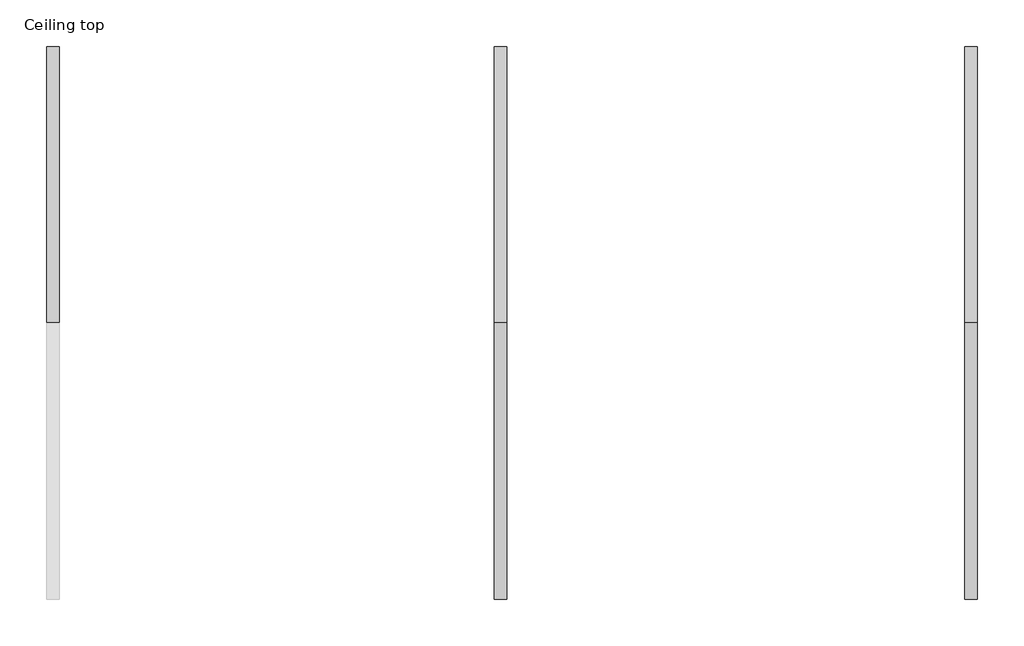
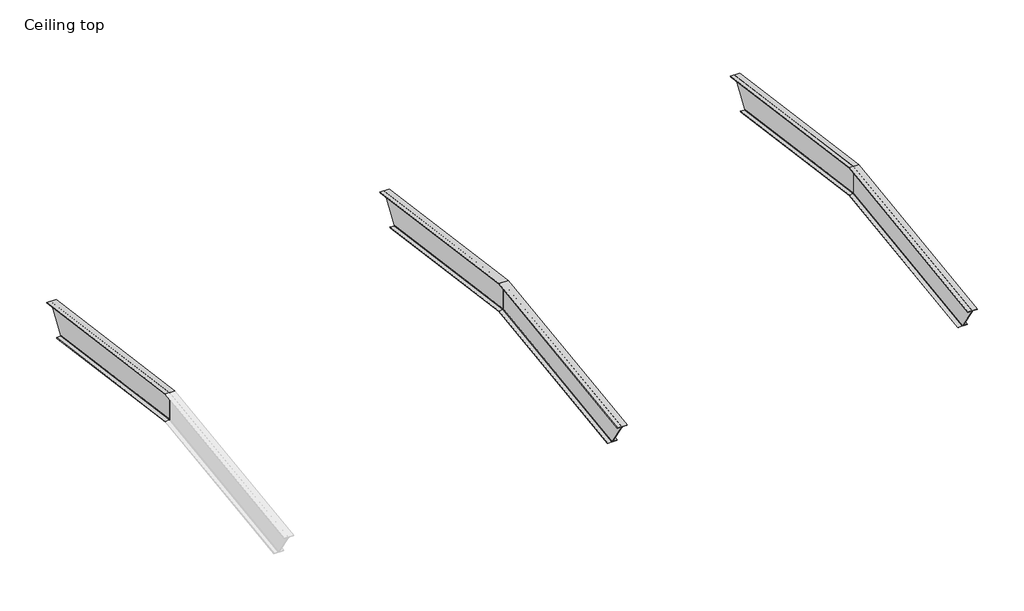
# One storey, part 2 of 2: 5 beams.
"""IFC4 building model written with IfcOpenShell, lengths in millimetres."""

from ifc_helpers import new_model, si_unit, frame, origin, place, context, project, spatial, polyline, ellipse_curve, element, save
from ifc_brep_helpers import plane_surface, revolved_surface, advanced_brep

model = new_model("IFC4")

# Units and contexts
model_context = context("Model", 3, world=origin())
ifc_project = project(units=[si_unit("LENGTHUNIT", "METRE", prefix="MILLI")], contexts=[model_context])

# Site, building, storey
site = spatial("IfcSite", under=ifc_project)
building = spatial("IfcBuilding", under=site)
storey = spatial("IfcBuildingStorey", under=building, Name="Ceiling top", Elevation=4718.05)

# Beams
placement = place(None, origin())
element("IfcBeam", 1, ObjectType="W Shapes : W 6X18.5", at=placement, inside=storey, context=model_context, shape_type="AdvancedBrep", body=[
    advanced_brep(
    [(28967.3280052, 7113.2615366, 4727.7884676), (29032.9870052, 7113.2615366, 4727.7884676), (29032.9870052, 10139.0601337, 4314.3781499), (28967.3280052, 10139.0601337, 4314.3781499), (28959.7080052, 7113.2615366, 4735.4792613), (28959.7080052, 10143.6843616, 4321.4371423), (28959.7080052, 7113.2615366, 5174.8799434), (28959.7080052, 10407.8819145, 4724.7409096), (28967.3280052, 7113.2615366, 5182.5707371), (28967.3280052, 10412.5061424, 4731.799902), (29032.9870052, 7113.2615366, 5182.5707371), (29032.9870052, 10412.5061424, 4731.799902), (29032.9870052, 7113.2615366, 5192.3124092), (29032.9870052, 10418.3634977, 4740.7412924), (28880.5870052, 7113.2615366, 5192.3124092), (28880.5870052, 10418.3634977, 4740.7412924), (28880.5870052, 7113.2615366, 5182.5707371), (28880.5870052, 10412.5061424, 4731.799902), (28946.2460052, 7113.2615366, 5182.5707371), (28946.2460052, 10412.5061424, 4731.799902), (28953.8660052, 7113.2615366, 5174.8799434), (28953.8660052, 10407.8819145, 4724.7409096), (28953.8660052, 7113.2615366, 4735.4792613), (28953.8660052, 10143.6843616, 4321.4371423), (28946.2460052, 7113.2615366, 4727.7884676), (28946.2460052, 10139.0601337, 4314.3781499), (28880.5870052, 7113.2615366, 4727.7884676), (28880.5870052, 10139.0601337, 4314.3781499), (28880.5870052, 7113.2615366, 4718.0467955), (28880.5870052, 10133.2027784, 4305.4367595), (29032.9870052, 7113.2615366, 4718.0467955), (29032.9870052, 10133.2027784, 4305.4367595)],
    [
        (0, 1),
        (1, 2),
        (2, 3),
        (3, 0),
        (4, 0, ellipse_curve(frame((28967.3280052, 7113.2615366, 4735.4792613), z_axis=(0.0, -1.0, 0.0), x_axis=(0.0, 0.0, -1.0)), 7.6907937, 7.62)),
        (3, 5, ellipse_curve(frame((28967.3280052, 10143.6843616, 4321.4371423), z_axis=(0.0, 0.836495308057375, -0.5479740866117643), x_axis=(0.0, 0.547974086611764, 0.8364953080573752)), 8.4387711, 7.62)),
        (5, 4),
        (6, 4),
        (5, 7),
        (7, 6),
        (8, 6, ellipse_curve(frame((28967.3280052, 7113.2615366, 5174.8799434), z_axis=(0.0, -1.0, 0.0), x_axis=(0.0, 0.0, -1.0)), 7.6907937, 7.62)),
        (7, 9, ellipse_curve(frame((28967.3280052, 10407.8819145, 4724.7409096), z_axis=(0.0, 0.836495308057375, -0.5479740866117643), x_axis=(0.0, 0.547974086611764, 0.8364953080573752)), 8.4387711, 7.62)),
        (9, 8),
        (10, 8),
        (9, 11),
        (11, 10),
        (12, 10),
        (11, 13),
        (13, 12),
        (14, 12),
        (13, 15),
        (15, 14),
        (16, 14),
        (15, 17),
        (17, 16),
        (18, 16),
        (17, 19),
        (19, 18),
        (20, 18, ellipse_curve(frame((28946.2460052, 7113.2615366, 5174.8799434), z_axis=(0.0, -1.0, 0.0), x_axis=(0.0, 0.0, -1.0)), 7.6907937, 7.62)),
        (19, 21, ellipse_curve(frame((28946.2460052, 10407.8819145, 4724.7409096), z_axis=(0.0, 0.836495308057375, -0.5479740866117643), x_axis=(0.0, 0.547974086611764, 0.8364953080573752)), 8.4387711, 7.62)),
        (21, 20),
        (22, 20),
        (21, 23),
        (23, 22),
        (24, 22, ellipse_curve(frame((28946.2460052, 7113.2615366, 4735.4792613), z_axis=(0.0, -1.0, 0.0), x_axis=(0.0, 0.0, -1.0)), 7.6907937, 7.62)),
        (23, 25, ellipse_curve(frame((28946.2460052, 10143.6843616, 4321.4371423), z_axis=(0.0, 0.836495308057375, -0.5479740866117643), x_axis=(0.0, 0.547974086611764, 0.8364953080573752)), 8.4387711, 7.62)),
        (25, 24),
        (26, 24),
        (25, 27),
        (27, 26),
        (28, 26),
        (27, 29),
        (29, 28),
        (30, 28),
        (29, 31),
        (31, 30),
        (1, 30),
        (31, 2),
    ],
    [
        plane_surface(frame((29032.9870052, 7050.9569516, 4736.3010494), z_axis=(0.0, 0.1353708330841357, 0.9907950027882191), x_axis=(0.0, 0.9907950027882191, -0.1353708330841357))),
        revolved_surface(polyline([(28959.708005200002, 10147.277063747912, 4320.946276885532), (28959.708005200002, 7112.230010863546, 4735.620197164001)]), (28967.3280052, 7051.9884774, 4743.8509074), (0.0, 0.9907950027882191, -0.1353708330841357)),
        plane_surface(frame((28959.7080052, 7051.9884774, 4743.8509074), z_axis=(1.0, 0.0, 0.0), x_axis=(0.0, 0.9907950027882191, -0.1353708330841357))),
        revolved_surface(polyline([(28959.708005200002, 10411.474616650441, 4724.25004406808), (28959.708005200002, 7112.230010852571, 5175.020879183669)]), (28967.3280052, 7110.9229818, 5175.1994566), (0.0, 0.9907950027882191, -0.1353708330841357)),
        plane_surface(frame((28967.3280052, 7111.9545075, 5182.7493145), z_axis=(0.0, -0.1353708330841357, -0.9907950027882191), x_axis=(0.0, 0.9907950027882191, -0.1353708330841357))),
        plane_surface(frame((29032.9870052, 7111.9545075, 5182.7493145), z_axis=(1.0, 0.0, 0.0), x_axis=(0.0, 0.9907950027882191, -0.1353708330841357))),
        plane_surface(frame((29032.9870052, 7113.2611068, 5192.3124679), z_axis=(0.0, 0.1353708330841357, 0.9907950027882191), x_axis=(0.0, 0.9907950027882191, -0.1353708330841357))),
        plane_surface(frame((28880.5870052, 7113.2611068, 5192.3124679), z_axis=(-1.0, 0.0, 0.0), x_axis=(0.0, 0.9907950027882191, -0.1353708330841357))),
        plane_surface(frame((28880.5870052, 7111.9545075, 5182.7493145), z_axis=(0.0, -0.1353708330841357, -0.9907950027882191), x_axis=(0.0, 0.9907950027882191, -0.1353708330841357))),
        revolved_surface(polyline([(28938.6260052, 10411.474616650441, 4724.25004406808), (28938.6260052, 7112.230010852571, 5175.020879183669)]), (28946.2460052, 7110.9229818, 5175.1994566), (0.0, 0.9907950027882191, -0.1353708330841357)),
        plane_surface(frame((28953.8660052, 7110.9229818, 5175.1994566), z_axis=(-1.0, 0.0, 0.0), x_axis=(0.0, 0.9907950027882191, -0.1353708330841357))),
        revolved_surface(polyline([(28938.6260052, 10147.277063747912, 4320.946276885532), (28938.6260052, 7112.230010863546, 4735.620197164001)]), (28946.2460052, 7051.9884774, 4743.8509074), (0.0, 0.9907950027882191, -0.1353708330841357)),
        plane_surface(frame((28946.2460052, 7050.9569516, 4736.3010494), z_axis=(0.0, 0.1353708330841357, 0.9907950027882191), x_axis=(0.0, 0.9907950027882191, -0.1353708330841357))),
        plane_surface(frame((28880.5870052, 7050.9569516, 4736.3010494), z_axis=(-1.0, 0.0, 0.0), x_axis=(0.0, 0.9907950027882191, -0.1353708330841357))),
        plane_surface(frame((28880.5870052, 7049.6503524, 4726.7378961), z_axis=(0.0, -0.1353708330841357, -0.9907950027882191), x_axis=(0.0, 0.9907950027882191, -0.1353708330841357))),
        plane_surface(frame((29032.9870052, 7049.6503524, 4726.7378961), z_axis=(1.0, 0.0, 0.0), x_axis=(0.0, 0.9907950027882191, -0.1353708330841357))),
        plane_surface(frame((28956.7905771, 10418.3654245, 4740.7442336), z_axis=(0.0, 0.836495308057375, -0.5479740866117643), x_axis=(1.0, 0.0, 0.0))),
        plane_surface(frame((28956.7905771, 7113.2615366, 5192.3156137), z_axis=(0.0, -1.0, 0.0), x_axis=(0.0, 0.0, 1.0))),
    ],
    [
        (0, [[1, 2, 3, 4]]),
        (1, [[5, -4, 6, 7]]),
        (2, [[8, -7, 9, 10]]),
        (3, [[11, -10, 12, 13]]),
        (4, [[14, -13, 15, 16]]),
        (5, [[17, -16, 18, 19]]),
        (6, [[20, -19, 21, 22]]),
        (7, [[23, -22, 24, 25]]),
        (8, [[26, -25, 27, 28]]),
        (9, [[29, -28, 30, 31]]),
        (10, [[32, -31, 33, 34]]),
        (11, [[35, -34, 36, 37]]),
        (12, [[38, -37, 39, 40]]),
        (13, [[41, -40, 42, 43]]),
        (14, [[44, -43, 45, 46]]),
        (15, [[47, -46, 48, -2]]),
        (16, [[-48, -45, -42, -39, -36, -33, -30, -27, -24, -21, -18, -15, -12, -9, -6, -3]]),
        (17, [[-1, -5, -8, -11, -14, -17, -20, -23, -26, -29, -32, -35, -38, -41, -44, -47]]),
    ],
),
])
element("IfcBeam", 2, ObjectType="W Shapes : W 6X18.5", at=placement, inside=storey, context=model_context, shape_type="AdvancedBrep", body=[
    advanced_brep(
    [(28967.3280052, 4087.4629396, 4314.3781499), (29032.9870052, 4087.4629396, 4314.3781499), (29032.9870052, 7113.2615366, 4727.7884676), (28967.3280052, 7113.2615366, 4727.7884676), (28959.7080052, 4082.8387117, 4321.4371423), (28959.7080052, 7113.2615366, 4735.4792613), (28959.7080052, 3818.6411587, 4724.7409096), (28959.7080052, 7113.2615366, 5174.8799434), (28967.3280052, 3814.0169308, 4731.799902), (28967.3280052, 7113.2615366, 5182.5707371), (29032.9870052, 3814.0169308, 4731.799902), (29032.9870052, 7113.2615366, 5182.5707371), (29032.9870052, 3808.1595755, 4740.7412924), (29032.9870052, 7113.2615366, 5192.3124092), (28880.5870052, 3808.1595755, 4740.7412924), (28880.5870052, 7113.2615366, 5192.3124092), (28880.5870052, 3814.0169308, 4731.799902), (28880.5870052, 7113.2615366, 5182.5707371), (28946.2460052, 3814.0169308, 4731.799902), (28946.2460052, 7113.2615366, 5182.5707371), (28953.8660052, 3818.6411587, 4724.7409096), (28953.8660052, 7113.2615366, 5174.8799434), (28953.8660052, 4082.8387117, 4321.4371423), (28953.8660052, 7113.2615366, 4735.4792613), (28946.2460052, 4087.4629396, 4314.3781499), (28946.2460052, 7113.2615366, 4727.7884676), (28880.5870052, 4087.4629396, 4314.3781499), (28880.5870052, 7113.2615366, 4727.7884676), (28880.5870052, 4093.3202949, 4305.4367595), (28880.5870052, 7113.2615366, 4718.0467955), (29032.9870052, 4093.3202949, 4305.4367595), (29032.9870052, 7113.2615366, 4718.0467955)],
    [
        (0, 1),
        (1, 2),
        (2, 3),
        (3, 0),
        (4, 0, ellipse_curve(frame((28967.3280052, 4082.8387117, 4321.4371423), z_axis=(0.0, -0.8364953080573767, -0.5479740866117618), x_axis=(0.0, 0.5479740866117613, -0.8364953080573769)), 8.4387711, 7.62)),
        (3, 5, ellipse_curve(frame((28967.3280052, 7113.2615366, 4735.4792613), z_axis=(0.0, 1.0, 0.0), x_axis=(0.0, 0.0, 1.0)), 7.6907937, 7.62)),
        (5, 4),
        (6, 4),
        (5, 7),
        (7, 6),
        (8, 6, ellipse_curve(frame((28967.3280052, 3818.6411587, 4724.7409096), z_axis=(0.0, -0.8364953080573767, -0.5479740866117618), x_axis=(0.0, 0.5479740866117613, -0.8364953080573769)), 8.4387711, 7.62)),
        (7, 9, ellipse_curve(frame((28967.3280052, 7113.2615366, 5174.8799434), z_axis=(0.0, 1.0, 0.0), x_axis=(0.0, 0.0, 1.0)), 7.6907937, 7.62)),
        (9, 8),
        (10, 8),
        (9, 11),
        (11, 10),
        (12, 10),
        (11, 13),
        (13, 12),
        (14, 12),
        (13, 15),
        (15, 14),
        (16, 14),
        (15, 17),
        (17, 16),
        (18, 16),
        (17, 19),
        (19, 18),
        (20, 18, ellipse_curve(frame((28946.2460052, 3818.6411587, 4724.7409096), z_axis=(0.0, -0.8364953080573767, -0.5479740866117618), x_axis=(0.0, 0.5479740866117613, -0.8364953080573769)), 8.4387711, 7.62)),
        (19, 21, ellipse_curve(frame((28946.2460052, 7113.2615366, 5174.8799434), z_axis=(0.0, 1.0, 0.0), x_axis=(0.0, 0.0, 1.0)), 7.6907937, 7.62)),
        (21, 20),
        (22, 20),
        (21, 23),
        (23, 22),
        (24, 22, ellipse_curve(frame((28946.2460052, 4082.8387117, 4321.4371423), z_axis=(0.0, -0.8364953080573767, -0.5479740866117618), x_axis=(0.0, 0.5479740866117613, -0.8364953080573769)), 8.4387711, 7.62)),
        (23, 25, ellipse_curve(frame((28946.2460052, 7113.2615366, 4735.4792613), z_axis=(0.0, 1.0, 0.0), x_axis=(0.0, 0.0, 1.0)), 7.6907937, 7.62)),
        (25, 24),
        (26, 24),
        (25, 27),
        (27, 26),
        (28, 26),
        (27, 29),
        (29, 28),
        (30, 28),
        (29, 31),
        (31, 30),
        (1, 30),
        (31, 2),
    ],
    [
        plane_surface(frame((29032.9870052, 3870.4622337, 4284.7296694), z_axis=(0.0, -0.13537083308413533, 0.9907950027882192), x_axis=(0.0, 0.9907950027882192, 0.13537083308413533))),
        revolved_surface(polyline([(28959.708005200002, 7114.293062347846, 4735.620197080616), (28959.708005200002, 4079.246009561649, 4320.946276815561)]), (28967.3280052, 3869.430708, 4292.2795273), (0.0, 0.9907950027882191, 0.1353708330841353)),
        plane_surface(frame((28959.7080052, 3869.430708, 4292.2795273), z_axis=(1.0, 0.0, 0.0), x_axis=(0.0, 0.9907950027882192, 0.13537083308413533))),
        revolved_surface(polyline([(28959.708005200002, 7114.293062345409, 5175.020879198452), (28959.708005200002, 3815.0484565475394, 4724.2500440828635)]), (28967.3280052, 3810.4962036, 4723.6280766), (0.0, 0.9907950027882191, 0.1353708330841353)),
        plane_surface(frame((28967.3280052, 3809.4646778, 4731.1779345), z_axis=(0.0, 0.13537083308413533, -0.9907950027882192), x_axis=(0.0, 0.9907950027882192, 0.13537083308413533))),
        plane_surface(frame((29032.9870052, 3809.4646778, 4731.1779345), z_axis=(1.0, 0.0, 0.0), x_axis=(0.0, 0.9907950027882192, 0.13537083308413533))),
        plane_surface(frame((29032.9870052, 3808.1580786, 4740.7410879), z_axis=(0.0, -0.13537083308413533, 0.9907950027882192), x_axis=(0.0, 0.9907950027882192, 0.13537083308413533))),
        plane_surface(frame((28880.5870052, 3808.1580786, 4740.7410879), z_axis=(-1.0, 0.0, 0.0), x_axis=(0.0, 0.9907950027882192, 0.13537083308413533))),
        plane_surface(frame((28880.5870052, 3809.4646778, 4731.1779345), z_axis=(0.0, 0.13537083308413533, -0.9907950027882192), x_axis=(0.0, 0.9907950027882192, 0.13537083308413533))),
        revolved_surface(polyline([(28938.6260052, 7114.293062345409, 5175.020879198452), (28938.6260052, 3815.0484565475394, 4724.2500440828635)]), (28946.2460052, 3810.4962036, 4723.6280766), (0.0, 0.9907950027882191, 0.1353708330841353)),
        plane_surface(frame((28953.8660052, 3810.4962036, 4723.6280766), z_axis=(-1.0, 0.0, 0.0), x_axis=(0.0, 0.9907950027882192, 0.13537083308413533))),
        revolved_surface(polyline([(28938.6260052, 7114.293062347846, 4735.620197080616), (28938.6260052, 4079.246009561649, 4320.946276815561)]), (28946.2460052, 3869.430708, 4292.2795273), (0.0, 0.9907950027882191, 0.1353708330841353)),
        plane_surface(frame((28946.2460052, 3870.4622337, 4284.7296694), z_axis=(0.0, -0.13537083308413533, 0.9907950027882192), x_axis=(0.0, 0.9907950027882192, 0.13537083308413533))),
        plane_surface(frame((28880.5870052, 3870.4622337, 4284.7296694), z_axis=(-1.0, 0.0, 0.0), x_axis=(0.0, 0.9907950027882192, 0.13537083308413533))),
        plane_surface(frame((28880.5870052, 3871.768833, 4275.166516), z_axis=(0.0, 0.13537083308413533, -0.9907950027882192), x_axis=(0.0, 0.9907950027882192, 0.13537083308413533))),
        plane_surface(frame((29032.9870052, 3871.768833, 4275.166516), z_axis=(1.0, 0.0, 0.0), x_axis=(0.0, 0.9907950027882192, 0.13537083308413533))),
        plane_surface(frame((28956.7905771, 7113.2615366, 5192.3156137), z_axis=(0.0, 1.0, 0.0), x_axis=(0.0, 0.0, -1.0))),
        plane_surface(frame((28956.7905771, 4093.3183681, 4305.4397008), z_axis=(0.0, -0.8364953080573767, -0.5479740866117618), x_axis=(1.0, 0.0, 0.0))),
    ],
    [
        (0, [[1, 2, 3, 4]]),
        (1, [[5, -4, 6, 7]]),
        (2, [[8, -7, 9, 10]]),
        (3, [[11, -10, 12, 13]]),
        (4, [[14, -13, 15, 16]]),
        (5, [[17, -16, 18, 19]]),
        (6, [[20, -19, 21, 22]]),
        (7, [[23, -22, 24, 25]]),
        (8, [[26, -25, 27, 28]]),
        (9, [[29, -28, 30, 31]]),
        (10, [[32, -31, 33, 34]]),
        (11, [[35, -34, 36, 37]]),
        (12, [[38, -37, 39, 40]]),
        (13, [[41, -40, 42, 43]]),
        (14, [[44, -43, 45, 46]]),
        (15, [[47, -46, 48, -2]]),
        (16, [[-48, -45, -42, -39, -36, -33, -30, -27, -24, -21, -18, -15, -12, -9, -6, -3]]),
        (17, [[-1, -5, -8, -11, -14, -17, -20, -23, -26, -29, -32, -35, -38, -41, -44, -47]]),
    ],
),
])
element("IfcBeam", 3, ObjectType="W Shapes : W 6X18.5", at=placement, inside=storey, context=model_context, shape_type="AdvancedBrep", body=[
    advanced_brep(
    [(23341.2280052, 7113.2615366, 4727.7884676), (23406.8870052, 7113.2615366, 4727.7884676), (23406.8870052, 10139.0601337, 4314.3781499), (23341.2280052, 10139.0601337, 4314.3781499), (23333.6080052, 7113.2615366, 4735.4792613), (23333.6080052, 10143.6843616, 4321.4371423), (23333.6080052, 7113.2615366, 5174.8799434), (23333.6080052, 10407.8819145, 4724.7409096), (23341.2280052, 7113.2615366, 5182.5707371), (23341.2280052, 10412.5061424, 4731.799902), (23406.8870052, 7113.2615366, 5182.5707371), (23406.8870052, 10412.5061424, 4731.799902), (23406.8870052, 7113.2615366, 5192.3124092), (23406.8870052, 10418.3634977, 4740.7412924), (23254.4870052, 7113.2615366, 5192.3124092), (23254.4870052, 10418.3634977, 4740.7412924), (23254.4870052, 7113.2615366, 5182.5707371), (23254.4870052, 10412.5061424, 4731.799902), (23320.1460052, 7113.2615366, 5182.5707371), (23320.1460052, 10412.5061424, 4731.799902), (23327.7660052, 7113.2615366, 5174.8799434), (23327.7660052, 10407.8819145, 4724.7409096), (23327.7660052, 7113.2615366, 4735.4792613), (23327.7660052, 10143.6843616, 4321.4371423), (23320.1460052, 7113.2615366, 4727.7884676), (23320.1460052, 10139.0601337, 4314.3781499), (23254.4870052, 7113.2615366, 4727.7884676), (23254.4870052, 10139.0601337, 4314.3781499), (23254.4870052, 7113.2615366, 4718.0467955), (23254.4870052, 10133.2027784, 4305.4367595), (23406.8870052, 7113.2615366, 4718.0467955), (23406.8870052, 10133.2027784, 4305.4367595)],
    [
        (0, 1),
        (1, 2),
        (2, 3),
        (3, 0),
        (4, 0, ellipse_curve(frame((23341.2280052, 7113.2615366, 4735.4792613), z_axis=(0.0, -1.0, 0.0), x_axis=(0.0, 0.0, -1.0)), 7.6907937, 7.62)),
        (3, 5, ellipse_curve(frame((23341.2280052, 10143.6843616, 4321.4371423), z_axis=(0.0, 0.836495308057375, -0.5479740866117643), x_axis=(0.0, 0.547974086611764, 0.8364953080573752)), 8.4387711, 7.62)),
        (5, 4),
        (6, 4),
        (5, 7),
        (7, 6),
        (8, 6, ellipse_curve(frame((23341.2280052, 7113.2615366, 5174.8799434), z_axis=(0.0, -1.0, 0.0), x_axis=(0.0, 0.0, -1.0)), 7.6907937, 7.62)),
        (7, 9, ellipse_curve(frame((23341.2280052, 10407.8819145, 4724.7409096), z_axis=(0.0, 0.836495308057375, -0.5479740866117643), x_axis=(0.0, 0.547974086611764, 0.8364953080573752)), 8.4387711, 7.62)),
        (9, 8),
        (10, 8),
        (9, 11),
        (11, 10),
        (12, 10),
        (11, 13),
        (13, 12),
        (14, 12),
        (13, 15),
        (15, 14),
        (16, 14),
        (15, 17),
        (17, 16),
        (18, 16),
        (17, 19),
        (19, 18),
        (20, 18, ellipse_curve(frame((23320.1460052, 7113.2615366, 5174.8799434), z_axis=(0.0, -1.0, 0.0), x_axis=(0.0, 0.0, -1.0)), 7.6907937, 7.62)),
        (19, 21, ellipse_curve(frame((23320.1460052, 10407.8819145, 4724.7409096), z_axis=(0.0, 0.836495308057375, -0.5479740866117643), x_axis=(0.0, 0.547974086611764, 0.8364953080573752)), 8.4387711, 7.62)),
        (21, 20),
        (22, 20),
        (21, 23),
        (23, 22),
        (24, 22, ellipse_curve(frame((23320.1460052, 7113.2615366, 4735.4792613), z_axis=(0.0, -1.0, 0.0), x_axis=(0.0, 0.0, -1.0)), 7.6907937, 7.62)),
        (23, 25, ellipse_curve(frame((23320.1460052, 10143.6843616, 4321.4371423), z_axis=(0.0, 0.836495308057375, -0.5479740866117643), x_axis=(0.0, 0.547974086611764, 0.8364953080573752)), 8.4387711, 7.62)),
        (25, 24),
        (26, 24),
        (25, 27),
        (27, 26),
        (28, 26),
        (27, 29),
        (29, 28),
        (30, 28),
        (29, 31),
        (31, 30),
        (1, 30),
        (31, 2),
    ],
    [
        plane_surface(frame((23406.8870052, 7050.9569516, 4736.3010494), z_axis=(0.0, 0.1353708330841357, 0.9907950027882191), x_axis=(0.0, 0.9907950027882191, -0.1353708330841357))),
        revolved_surface(polyline([(23333.6080052, 10147.277063747912, 4320.946276885532), (23333.6080052, 7112.230010863546, 4735.620197164001)]), (23341.2280052, 7051.9884774, 4743.8509074), (0.0, 0.9907950027882191, -0.1353708330841357)),
        plane_surface(frame((23333.6080052, 7051.9884774, 4743.8509074), z_axis=(1.0, 0.0, 0.0), x_axis=(0.0, 0.9907950027882191, -0.1353708330841357))),
        revolved_surface(polyline([(23333.6080052, 10411.474616650441, 4724.25004406808), (23333.6080052, 7112.230010852571, 5175.020879183669)]), (23341.2280052, 7110.9229818, 5175.1994566), (0.0, 0.9907950027882191, -0.1353708330841357)),
        plane_surface(frame((23341.2280052, 7111.9545075, 5182.7493145), z_axis=(0.0, -0.1353708330841357, -0.9907950027882191), x_axis=(0.0, 0.9907950027882191, -0.1353708330841357))),
        plane_surface(frame((23406.8870052, 7111.9545075, 5182.7493145), z_axis=(1.0, 0.0, 0.0), x_axis=(0.0, 0.9907950027882191, -0.1353708330841357))),
        plane_surface(frame((23406.8870052, 7113.2611068, 5192.3124679), z_axis=(0.0, 0.1353708330841357, 0.9907950027882191), x_axis=(0.0, 0.9907950027882191, -0.1353708330841357))),
        plane_surface(frame((23254.4870052, 7113.2611068, 5192.3124679), z_axis=(-1.0, 0.0, 0.0), x_axis=(0.0, 0.9907950027882191, -0.1353708330841357))),
        plane_surface(frame((23254.4870052, 7111.9545075, 5182.7493145), z_axis=(0.0, -0.1353708330841357, -0.9907950027882191), x_axis=(0.0, 0.9907950027882191, -0.1353708330841357))),
        revolved_surface(polyline([(23312.5260052, 10411.474616650441, 4724.25004406808), (23312.5260052, 7112.230010852571, 5175.020879183669)]), (23320.1460052, 7110.9229818, 5175.1994566), (0.0, 0.9907950027882191, -0.1353708330841357)),
        plane_surface(frame((23327.7660052, 7110.9229818, 5175.1994566), z_axis=(-1.0, 0.0, 0.0), x_axis=(0.0, 0.9907950027882191, -0.1353708330841357))),
        revolved_surface(polyline([(23312.5260052, 10147.277063747912, 4320.946276885532), (23312.5260052, 7112.230010863546, 4735.620197164001)]), (23320.1460052, 7051.9884774, 4743.8509074), (0.0, 0.9907950027882191, -0.1353708330841357)),
        plane_surface(frame((23320.1460052, 7050.9569516, 4736.3010494), z_axis=(0.0, 0.1353708330841357, 0.9907950027882191), x_axis=(0.0, 0.9907950027882191, -0.1353708330841357))),
        plane_surface(frame((23254.4870052, 7050.9569516, 4736.3010494), z_axis=(-1.0, 0.0, 0.0), x_axis=(0.0, 0.9907950027882191, -0.1353708330841357))),
        plane_surface(frame((23254.4870052, 7049.6503524, 4726.7378961), z_axis=(0.0, -0.1353708330841357, -0.9907950027882191), x_axis=(0.0, 0.9907950027882191, -0.1353708330841357))),
        plane_surface(frame((23406.8870052, 7049.6503524, 4726.7378961), z_axis=(1.0, 0.0, 0.0), x_axis=(0.0, 0.9907950027882191, -0.1353708330841357))),
        plane_surface(frame((23330.6905771, 7113.2615366, 5192.3156137), z_axis=(0.0, -1.0, 0.0), x_axis=(0.0, 0.0, 1.0))),
        plane_surface(frame((23330.6905771, 10418.3654245, 4740.7442336), z_axis=(0.0, 0.836495308057375, -0.5479740866117643), x_axis=(1.0, 0.0, 0.0))),
    ],
    [
        (0, [[1, 2, 3, 4]]),
        (1, [[5, -4, 6, 7]]),
        (2, [[8, -7, 9, 10]]),
        (3, [[11, -10, 12, 13]]),
        (4, [[14, -13, 15, 16]]),
        (5, [[17, -16, 18, 19]]),
        (6, [[20, -19, 21, 22]]),
        (7, [[23, -22, 24, 25]]),
        (8, [[26, -25, 27, 28]]),
        (9, [[29, -28, 30, 31]]),
        (10, [[32, -31, 33, 34]]),
        (11, [[35, -34, 36, 37]]),
        (12, [[38, -37, 39, 40]]),
        (13, [[41, -40, 42, 43]]),
        (14, [[44, -43, 45, 46]]),
        (15, [[47, -46, 48, -2]]),
        (16, [[-1, -5, -8, -11, -14, -17, -20, -23, -26, -29, -32, -35, -38, -41, -44, -47]]),
        (17, [[-48, -45, -42, -39, -36, -33, -30, -27, -24, -21, -18, -15, -12, -9, -6, -3]]),
    ],
),
])
element("IfcBeam", 4, ObjectType="W Shapes : W 6X18.5", at=placement, inside=storey, context=model_context, shape_type="AdvancedBrep", body=[
    advanced_brep(
    [(23341.2280052, 4087.4629396, 4314.3781499), (23406.8870052, 4087.4629396, 4314.3781499), (23406.8870052, 7113.2615366, 4727.7884676), (23341.2280052, 7113.2615366, 4727.7884676), (23333.6080052, 4082.8387117, 4321.4371423), (23333.6080052, 7113.2615366, 4735.4792613), (23333.6080052, 3818.6411587, 4724.7409096), (23333.6080052, 7113.2615366, 5174.8799434), (23341.2280052, 3814.0169308, 4731.799902), (23341.2280052, 7113.2615366, 5182.5707371), (23406.8870052, 3814.0169308, 4731.799902), (23406.8870052, 7113.2615366, 5182.5707371), (23406.8870052, 3808.1595755, 4740.7412924), (23406.8870052, 7113.2615366, 5192.3124092), (23254.4870052, 3808.1595755, 4740.7412924), (23254.4870052, 7113.2615366, 5192.3124092), (23254.4870052, 3814.0169308, 4731.799902), (23254.4870052, 7113.2615366, 5182.5707371), (23320.1460052, 3814.0169308, 4731.799902), (23320.1460052, 7113.2615366, 5182.5707371), (23327.7660052, 3818.6411587, 4724.7409096), (23327.7660052, 7113.2615366, 5174.8799434), (23327.7660052, 4082.8387117, 4321.4371423), (23327.7660052, 7113.2615366, 4735.4792613), (23320.1460052, 4087.4629396, 4314.3781499), (23320.1460052, 7113.2615366, 4727.7884676), (23254.4870052, 4087.4629396, 4314.3781499), (23254.4870052, 7113.2615366, 4727.7884676), (23254.4870052, 4093.3202949, 4305.4367595), (23254.4870052, 7113.2615366, 4718.0467955), (23406.8870052, 4093.3202949, 4305.4367595), (23406.8870052, 7113.2615366, 4718.0467955)],
    [
        (0, 1),
        (1, 2),
        (2, 3),
        (3, 0),
        (4, 0, ellipse_curve(frame((23341.2280052, 4082.8387117, 4321.4371423), z_axis=(0.0, -0.8364953080573767, -0.5479740866117618), x_axis=(0.0, 0.5479740866117613, -0.8364953080573769)), 8.4387711, 7.62)),
        (3, 5, ellipse_curve(frame((23341.2280052, 7113.2615366, 4735.4792613), z_axis=(0.0, 1.0, 0.0), x_axis=(0.0, 0.0, 1.0)), 7.6907937, 7.62)),
        (5, 4),
        (6, 4),
        (5, 7),
        (7, 6),
        (8, 6, ellipse_curve(frame((23341.2280052, 3818.6411587, 4724.7409096), z_axis=(0.0, -0.8364953080573767, -0.5479740866117618), x_axis=(0.0, 0.5479740866117613, -0.8364953080573769)), 8.4387711, 7.62)),
        (7, 9, ellipse_curve(frame((23341.2280052, 7113.2615366, 5174.8799434), z_axis=(0.0, 1.0, 0.0), x_axis=(0.0, 0.0, 1.0)), 7.6907937, 7.62)),
        (9, 8),
        (10, 8),
        (9, 11),
        (11, 10),
        (12, 10),
        (11, 13),
        (13, 12),
        (14, 12),
        (13, 15),
        (15, 14),
        (16, 14),
        (15, 17),
        (17, 16),
        (18, 16),
        (17, 19),
        (19, 18),
        (20, 18, ellipse_curve(frame((23320.1460052, 3818.6411587, 4724.7409096), z_axis=(0.0, -0.8364953080573767, -0.5479740866117618), x_axis=(0.0, 0.5479740866117613, -0.8364953080573769)), 8.4387711, 7.62)),
        (19, 21, ellipse_curve(frame((23320.1460052, 7113.2615366, 5174.8799434), z_axis=(0.0, 1.0, 0.0), x_axis=(0.0, 0.0, 1.0)), 7.6907937, 7.62)),
        (21, 20),
        (22, 20),
        (21, 23),
        (23, 22),
        (24, 22, ellipse_curve(frame((23320.1460052, 4082.8387117, 4321.4371423), z_axis=(0.0, -0.8364953080573767, -0.5479740866117618), x_axis=(0.0, 0.5479740866117613, -0.8364953080573769)), 8.4387711, 7.62)),
        (23, 25, ellipse_curve(frame((23320.1460052, 7113.2615366, 4735.4792613), z_axis=(0.0, 1.0, 0.0), x_axis=(0.0, 0.0, 1.0)), 7.6907937, 7.62)),
        (25, 24),
        (26, 24),
        (25, 27),
        (27, 26),
        (28, 26),
        (27, 29),
        (29, 28),
        (30, 28),
        (29, 31),
        (31, 30),
        (1, 30),
        (31, 2),
    ],
    [
        plane_surface(frame((23406.8870052, 3870.4622337, 4284.7296694), z_axis=(0.0, -0.13537083308413533, 0.9907950027882192), x_axis=(0.0, 0.9907950027882192, 0.13537083308413533))),
        revolved_surface(polyline([(23333.6080052, 7114.293062347846, 4735.620197080616), (23333.6080052, 4079.246009561649, 4320.946276815561)]), (23341.2280052, 3869.430708, 4292.2795273), (0.0, 0.9907950027882191, 0.1353708330841353)),
        plane_surface(frame((23333.6080052, 3869.430708, 4292.2795273), z_axis=(1.0, 0.0, 0.0), x_axis=(0.0, 0.9907950027882192, 0.13537083308413533))),
        revolved_surface(polyline([(23333.6080052, 7114.293062345409, 5175.020879198452), (23333.6080052, 3815.0484565475394, 4724.2500440828635)]), (23341.2280052, 3810.4962036, 4723.6280766), (0.0, 0.9907950027882191, 0.1353708330841353)),
        plane_surface(frame((23341.2280052, 3809.4646778, 4731.1779345), z_axis=(0.0, 0.13537083308413533, -0.9907950027882192), x_axis=(0.0, 0.9907950027882192, 0.13537083308413533))),
        plane_surface(frame((23406.8870052, 3809.4646778, 4731.1779345), z_axis=(1.0, 0.0, 0.0), x_axis=(0.0, 0.9907950027882192, 0.13537083308413533))),
        plane_surface(frame((23406.8870052, 3808.1580786, 4740.7410879), z_axis=(0.0, -0.13537083308413533, 0.9907950027882192), x_axis=(0.0, 0.9907950027882192, 0.13537083308413533))),
        plane_surface(frame((23254.4870052, 3808.1580786, 4740.7410879), z_axis=(-1.0, 0.0, 0.0), x_axis=(0.0, 0.9907950027882192, 0.13537083308413533))),
        plane_surface(frame((23254.4870052, 3809.4646778, 4731.1779345), z_axis=(0.0, 0.13537083308413533, -0.9907950027882192), x_axis=(0.0, 0.9907950027882192, 0.13537083308413533))),
        revolved_surface(polyline([(23312.5260052, 7114.293062345409, 5175.020879198452), (23312.5260052, 3815.0484565475394, 4724.2500440828635)]), (23320.1460052, 3810.4962036, 4723.6280766), (0.0, 0.9907950027882191, 0.1353708330841353)),
        plane_surface(frame((23327.7660052, 3810.4962036, 4723.6280766), z_axis=(-1.0, 0.0, 0.0), x_axis=(0.0, 0.9907950027882192, 0.13537083308413533))),
        revolved_surface(polyline([(23312.5260052, 7114.293062347846, 4735.620197080616), (23312.5260052, 4079.246009561649, 4320.946276815561)]), (23320.1460052, 3869.430708, 4292.2795273), (0.0, 0.9907950027882191, 0.1353708330841353)),
        plane_surface(frame((23320.1460052, 3870.4622337, 4284.7296694), z_axis=(0.0, -0.13537083308413533, 0.9907950027882192), x_axis=(0.0, 0.9907950027882192, 0.13537083308413533))),
        plane_surface(frame((23254.4870052, 3870.4622337, 4284.7296694), z_axis=(-1.0, 0.0, 0.0), x_axis=(0.0, 0.9907950027882192, 0.13537083308413533))),
        plane_surface(frame((23254.4870052, 3871.768833, 4275.166516), z_axis=(0.0, 0.13537083308413533, -0.9907950027882192), x_axis=(0.0, 0.9907950027882192, 0.13537083308413533))),
        plane_surface(frame((23406.8870052, 3871.768833, 4275.166516), z_axis=(1.0, 0.0, 0.0), x_axis=(0.0, 0.9907950027882192, 0.13537083308413533))),
        plane_surface(frame((23330.6905771, 7113.2615366, 5192.3156137), z_axis=(0.0, 1.0, 0.0), x_axis=(0.0, 0.0, -1.0))),
        plane_surface(frame((23330.6905771, 4093.3183681, 4305.4397008), z_axis=(0.0, -0.8364953080573767, -0.5479740866117618), x_axis=(1.0, 0.0, 0.0))),
    ],
    [
        (0, [[1, 2, 3, 4]]),
        (1, [[5, -4, 6, 7]]),
        (2, [[8, -7, 9, 10]]),
        (3, [[11, -10, 12, 13]]),
        (4, [[14, -13, 15, 16]]),
        (5, [[17, -16, 18, 19]]),
        (6, [[20, -19, 21, 22]]),
        (7, [[23, -22, 24, 25]]),
        (8, [[26, -25, 27, 28]]),
        (9, [[29, -28, 30, 31]]),
        (10, [[32, -31, 33, 34]]),
        (11, [[35, -34, 36, 37]]),
        (12, [[38, -37, 39, 40]]),
        (13, [[41, -40, 42, 43]]),
        (14, [[44, -43, 45, 46]]),
        (15, [[47, -46, 48, -2]]),
        (16, [[-48, -45, -42, -39, -36, -33, -30, -27, -24, -21, -18, -15, -12, -9, -6, -3]]),
        (17, [[-1, -5, -8, -11, -14, -17, -20, -23, -26, -29, -32, -35, -38, -41, -44, -47]]),
    ],
),
])
element("IfcBeam", 5, ObjectType="W Shapes : W 6X18.5", at=placement, inside=storey, context=model_context, shape_type="AdvancedBrep", body=[
    advanced_brep(
    [(17988.1780052, 7113.2615366, 4727.7884676), (18053.8370052, 7113.2615366, 4727.7884676), (18053.8370052, 10139.0601337, 4314.3781499), (17988.1780052, 10139.0601337, 4314.3781499), (17980.5580052, 7113.2615366, 4735.4792613), (17980.5580052, 10143.6843616, 4321.4371423), (17980.5580052, 7113.2615366, 5174.8799434), (17980.5580052, 10407.8819145, 4724.7409096), (17988.1780052, 7113.2615366, 5182.5707371), (17988.1780052, 10412.5061424, 4731.799902), (18053.8370052, 7113.2615366, 5182.5707371), (18053.8370052, 10412.5061424, 4731.799902), (18053.8370052, 7113.2615366, 5192.3124092), (18053.8370052, 10418.3634977, 4740.7412924), (17901.4370052, 7113.2615366, 5192.3124092), (17901.4370052, 10418.3634977, 4740.7412924), (17901.4370052, 7113.2615366, 5182.5707371), (17901.4370052, 10412.5061424, 4731.799902), (17967.0960052, 7113.2615366, 5182.5707371), (17967.0960052, 10412.5061424, 4731.799902), (17974.7160052, 7113.2615366, 5174.8799434), (17974.7160052, 10407.8819145, 4724.7409096), (17974.7160052, 7113.2615366, 4735.4792613), (17974.7160052, 10143.6843616, 4321.4371423), (17967.0960052, 7113.2615366, 4727.7884676), (17967.0960052, 10139.0601337, 4314.3781499), (17901.4370052, 7113.2615366, 4727.7884676), (17901.4370052, 10139.0601337, 4314.3781499), (17901.4370052, 7113.2615366, 4718.0467955), (17901.4370052, 10133.2027784, 4305.4367595), (18053.8370052, 7113.2615366, 4718.0467955), (18053.8370052, 10133.2027784, 4305.4367595)],
    [
        (0, 1),
        (1, 2),
        (2, 3),
        (3, 0),
        (4, 0, ellipse_curve(frame((17988.1780052, 7113.2615366, 4735.4792613), z_axis=(0.0, -1.0, 0.0), x_axis=(0.0, 0.0, -1.0)), 7.6907937, 7.62)),
        (3, 5, ellipse_curve(frame((17988.1780052, 10143.6843616, 4321.4371423), z_axis=(0.0, 0.836495308057375, -0.5479740866117643), x_axis=(0.0, 0.547974086611764, 0.8364953080573752)), 8.4387711, 7.62)),
        (5, 4),
        (6, 4),
        (5, 7),
        (7, 6),
        (8, 6, ellipse_curve(frame((17988.1780052, 7113.2615366, 5174.8799434), z_axis=(0.0, -1.0, 0.0), x_axis=(0.0, 0.0, -1.0)), 7.6907937, 7.62)),
        (7, 9, ellipse_curve(frame((17988.1780052, 10407.8819145, 4724.7409096), z_axis=(0.0, 0.836495308057375, -0.5479740866117643), x_axis=(0.0, 0.547974086611764, 0.8364953080573752)), 8.4387711, 7.62)),
        (9, 8),
        (10, 8),
        (9, 11),
        (11, 10),
        (12, 10),
        (11, 13),
        (13, 12),
        (14, 12),
        (13, 15),
        (15, 14),
        (16, 14),
        (15, 17),
        (17, 16),
        (18, 16),
        (17, 19),
        (19, 18),
        (20, 18, ellipse_curve(frame((17967.0960052, 7113.2615366, 5174.8799434), z_axis=(0.0, -1.0, 0.0), x_axis=(0.0, 0.0, -1.0)), 7.6907937, 7.62)),
        (19, 21, ellipse_curve(frame((17967.0960052, 10407.8819145, 4724.7409096), z_axis=(0.0, 0.836495308057375, -0.5479740866117643), x_axis=(0.0, 0.547974086611764, 0.8364953080573752)), 8.4387711, 7.62)),
        (21, 20),
        (22, 20),
        (21, 23),
        (23, 22),
        (24, 22, ellipse_curve(frame((17967.0960052, 7113.2615366, 4735.4792613), z_axis=(0.0, -1.0, 0.0), x_axis=(0.0, 0.0, -1.0)), 7.6907937, 7.62)),
        (23, 25, ellipse_curve(frame((17967.0960052, 10143.6843616, 4321.4371423), z_axis=(0.0, 0.836495308057375, -0.5479740866117643), x_axis=(0.0, 0.547974086611764, 0.8364953080573752)), 8.4387711, 7.62)),
        (25, 24),
        (26, 24),
        (25, 27),
        (27, 26),
        (28, 26),
        (27, 29),
        (29, 28),
        (30, 28),
        (29, 31),
        (31, 30),
        (1, 30),
        (31, 2),
    ],
    [
        plane_surface(frame((18053.8370052, 7050.9569516, 4736.3010494), z_axis=(0.0, 0.1353708330841357, 0.9907950027882191), x_axis=(0.0, 0.9907950027882191, -0.1353708330841357))),
        revolved_surface(polyline([(17980.5580052, 10147.277063747912, 4320.946276885532), (17980.5580052, 7112.230010863546, 4735.620197164001)]), (17988.1780052, 7051.9884774, 4743.8509074), (0.0, 0.9907950027882191, -0.1353708330841357)),
        plane_surface(frame((17980.5580052, 7051.9884774, 4743.8509074), z_axis=(1.0, 0.0, 0.0), x_axis=(0.0, 0.9907950027882191, -0.1353708330841357))),
        revolved_surface(polyline([(17980.5580052, 10411.474616650441, 4724.25004406808), (17980.5580052, 7112.230010852571, 5175.020879183669)]), (17988.1780052, 7110.9229818, 5175.1994566), (0.0, 0.9907950027882191, -0.1353708330841357)),
        plane_surface(frame((17988.1780052, 7111.9545075, 5182.7493145), z_axis=(0.0, -0.1353708330841357, -0.9907950027882191), x_axis=(0.0, 0.9907950027882191, -0.1353708330841357))),
        plane_surface(frame((18053.8370052, 7111.9545075, 5182.7493145), z_axis=(1.0, 0.0, 0.0), x_axis=(0.0, 0.9907950027882191, -0.1353708330841357))),
        plane_surface(frame((18053.8370052, 7113.2611068, 5192.3124679), z_axis=(0.0, 0.1353708330841357, 0.9907950027882191), x_axis=(0.0, 0.9907950027882191, -0.1353708330841357))),
        plane_surface(frame((17901.4370052, 7113.2611068, 5192.3124679), z_axis=(-1.0, 0.0, 0.0), x_axis=(0.0, 0.9907950027882191, -0.1353708330841357))),
        plane_surface(frame((17901.4370052, 7111.9545075, 5182.7493145), z_axis=(0.0, -0.1353708330841357, -0.9907950027882191), x_axis=(0.0, 0.9907950027882191, -0.1353708330841357))),
        revolved_surface(polyline([(17959.476005200002, 10411.474616650441, 4724.25004406808), (17959.476005200002, 7112.230010852571, 5175.020879183669)]), (17967.0960052, 7110.9229818, 5175.1994566), (0.0, 0.9907950027882191, -0.1353708330841357)),
        plane_surface(frame((17974.7160052, 7110.9229818, 5175.1994566), z_axis=(-1.0, 0.0, 0.0), x_axis=(0.0, 0.9907950027882191, -0.1353708330841357))),
        revolved_surface(polyline([(17959.476005200002, 10147.277063747912, 4320.946276885532), (17959.476005200002, 7112.230010863546, 4735.620197164001)]), (17967.0960052, 7051.9884774, 4743.8509074), (0.0, 0.9907950027882191, -0.1353708330841357)),
        plane_surface(frame((17967.0960052, 7050.9569516, 4736.3010494), z_axis=(0.0, 0.1353708330841357, 0.9907950027882191), x_axis=(0.0, 0.9907950027882191, -0.1353708330841357))),
        plane_surface(frame((17901.4370052, 7050.9569516, 4736.3010494), z_axis=(-1.0, 0.0, 0.0), x_axis=(0.0, 0.9907950027882191, -0.1353708330841357))),
        plane_surface(frame((17901.4370052, 7049.6503524, 4726.7378961), z_axis=(0.0, -0.1353708330841357, -0.9907950027882191), x_axis=(0.0, 0.9907950027882191, -0.1353708330841357))),
        plane_surface(frame((18053.8370052, 7049.6503524, 4726.7378961), z_axis=(1.0, 0.0, 0.0), x_axis=(0.0, 0.9907950027882191, -0.1353708330841357))),
        plane_surface(frame((17977.6405771, 7113.2615366, 5192.3156137), z_axis=(0.0, -1.0, 0.0), x_axis=(0.0, 0.0, 1.0))),
        plane_surface(frame((17977.6405771, 10418.3654245, 4740.7442336), z_axis=(0.0, 0.836495308057375, -0.5479740866117643), x_axis=(1.0, 0.0, 0.0))),
    ],
    [
        (0, [[1, 2, 3, 4]]),
        (1, [[5, -4, 6, 7]]),
        (2, [[8, -7, 9, 10]]),
        (3, [[11, -10, 12, 13]]),
        (4, [[14, -13, 15, 16]]),
        (5, [[17, -16, 18, 19]]),
        (6, [[20, -19, 21, 22]]),
        (7, [[23, -22, 24, 25]]),
        (8, [[26, -25, 27, 28]]),
        (9, [[29, -28, 30, 31]]),
        (10, [[32, -31, 33, 34]]),
        (11, [[35, -34, 36, 37]]),
        (12, [[38, -37, 39, 40]]),
        (13, [[41, -40, 42, 43]]),
        (14, [[44, -43, 45, 46]]),
        (15, [[47, -46, 48, -2]]),
        (16, [[-1, -5, -8, -11, -14, -17, -20, -23, -26, -29, -32, -35, -38, -41, -44, -47]]),
        (17, [[-48, -45, -42, -39, -36, -33, -30, -27, -24, -21, -18, -15, -12, -9, -6, -3]]),
    ],
),
])

save(model, "model.ifc")

# Revit data of these elements
# Type "W Shapes : W 6X18.5"
#   Section Name Key = "W12x26"
#   Assembly Code = "B10"
#   Width = 152.4 mm
#   Web Thickness = 5.842 mm
#   Web Fillet = 7.62 mm
#   Warping Constant = 163001.3 cm⁶
#   Torsional Moment of Inertia = 12.4869 cm⁴
#   Section Area = 7.65 in²
#   Plastic Modulus weak axis = 0.00472801 (stored number, unit not read)
#   Plastic Modulus strong axis = 0.0215278 (stored number, unit not read)
#   Perimeter = 15.0571 m²/m
#   Nominal Weight = 379.441 N/m
#   Moment of Inertia weak axis = 720.08 cm⁴
#   Moment of Inertia strong axis = 8491.12 cm⁴
#   Height = 469.9 mm
#   Flange Thickness = 9.652 mm
#   Elastic Modulus weak axis = 0.00309028 (stored number, unit not read)
#   Elastic Modulus strong axis = 0.0193287 (stored number, unit not read)
#   Centroid Vertical = 234.95 mm
#   Centroid Horizontal = 76.2 mm
#   Length [instance default] = 5' - 0"
#   Structural Material [instance default] = Steel ASTM A992
#   Principal Axes Angle = 0
# Elements 1, 2, 3, 4, 5 (IfcBeam, "W Shapes : W 6X18.5")
#   Comments = ""
#   Structural Material = Steel ASTM A992
#   Phase Created = New Construction
#   Materials on its faces: "Steel ASTM A992"
# Materials
#   "Steel ASTM A992": class "Metal", colour RGB 189 187 185, transparency 0, Description = "Structural steel 50ksi", Cost = 0
